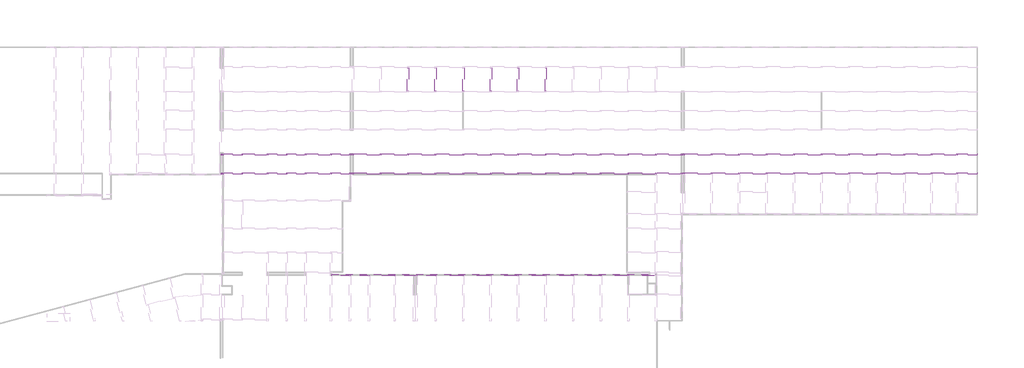
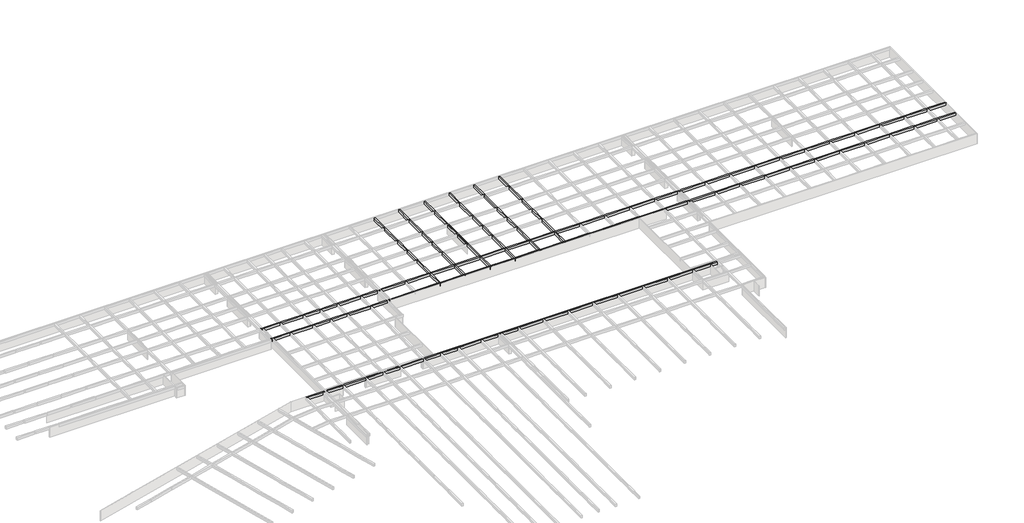
# One storey, part 11 of 14: 9 beams.
"""IFC4 building model written with IfcOpenShell, lengths in millimetres."""

from ifc_helpers import new_model, si_unit, frame, origin, place, context, project, spatial, polyline, outline, extrude, faceted_brep, element, save

model = new_model("IFC4")

# Units and contexts
model_context = context("Model", 3, world=origin())
ifc_project = project(units=[si_unit("LENGTHUNIT", "METRE", prefix="MILLI")], contexts=[model_context])

# Site, building, storey
site = spatial("IfcSite", under=ifc_project)
building = spatial("IfcBuilding", under=site)
storey = spatial("IfcBuildingStorey", under=building, Name="户型图", Elevation=0.0)

# Beams
placement = place(None, origin())
element("IfcBeam", 1, ObjectType="混凝土 - 矩形梁 : KL_beam", at=placement, inside=storey, context=model_context, shape_type="Brep", body=[
    faceted_brep([(227227.2949044, -147499.284307, 3300.0), (227227.2949044, -147899.284307, 3300.0), (227227.2949044, -147899.284307, 2500.0), (227227.2949044, -147499.284307, 2500.0), (221727.2949044, -147499.284307, 3300.0), (221327.2949044, -147499.284307, 3300.0), (214491.1566028, -147499.284307, 3300.0), (214091.1566028, -147499.284307, 3300.0), (206763.3308695, -147499.284307, 3300.0), (206363.3308695, -147499.284307, 3300.0), (198949.6658892, -147499.284307, 3300.0), (198549.6658892, -147499.284307, 3300.0), (191137.2949044, -147499.284307, 3300.0), (190737.2949044, -147499.284307, 3300.0), (183327.7006088, -147499.284307, 3300.0), (182927.7006088, -147499.284307, 3300.0), (175558.5232577, -147499.284307, 3300.0), (175158.5232577, -147499.284307, 3300.0), (167740.9658811, -147499.284307, 3300.0), (167340.9658811, -147499.284307, 3300.0), (159907.8874304, -147499.284307, 3300.0), (159507.8874304, -147499.284307, 3300.0), (152140.9658811, -147499.284307, 3300.0), (151740.9658811, -147499.284307, 3300.0), (144337.2949044, -147499.284307, 3300.0), (143937.2949044, -147499.284307, 3300.0), (143577.2949044, -147499.284307, 3300.0), (143177.2949044, -147499.284307, 3300.0), (136347.2949044, -147499.284307, 3300.0), (135947.2949044, -147499.284307, 3300.0), (128527.2949044, -147499.284307, 3300.0), (128127.2949044, -147499.284307, 3300.0), (120717.7893795, -147499.284307, 3300.0), (120317.7893795, -147499.284307, 3300.0), (112927.2949044, -147499.284307, 3300.0), (112527.2949044, -147499.284307, 3300.0), (105157.0968236, -147499.284307, 3300.0), (104757.0968236, -147499.284307, 3300.0), (97322.1026691, -147499.284307, 3300.0), (96922.1026691, -147499.284307, 3300.0), (89602.2949044, -147499.284307, 3300.0), (89202.2949044, -147499.284307, 3300.0), (81802.2949044, -147499.284307, 3300.0), (81402.2949044, -147499.284307, 3300.0), (73867.4871398, -147499.284307, 3300.0), (73467.4871398, -147499.284307, 3300.0), (66130.1134745, -147499.284307, 3300.0), (65730.1134745, -147499.284307, 3300.0), (58330.1134745, -147499.284307, 3300.0), (57930.1134745, -147499.284307, 3300.0), (50537.2949044, -147499.284307, 3300.0), (50137.2949044, -147499.284307, 3300.0), (49716.5330009, -147499.284307, 3300.0), (49316.5330009, -147499.284307, 3300.0), (44331.9066405, -147499.284307, 3300.0), (43931.9066405, -147499.284307, 3300.0), (37081.5607309, -147499.284307, 3300.0), (36681.5607309, -147499.284307, 3300.0), (31751.9066405, -147499.284307, 3300.0), (31351.9066405, -147499.284307, 3300.0), (26321.5607309, -147499.284307, 3300.0), (25921.5607309, -147499.284307, 3300.0), (19160.0865653, -147499.284307, 3300.0), (18760.0865653, -147499.284307, 3300.0), (13677.2949044, -147499.284307, 3300.0), (13277.2949044, -147499.284307, 3300.0), (12977.2949044, -147499.284307, 3300.0), (12977.2949044, -147899.284307, 3300.0), (13277.2949044, -147899.284307, 3300.0), (13677.2949044, -147899.284307, 3300.0), (18760.0865653, -147899.284307, 3300.0), (19160.0865653, -147899.284307, 3300.0), (25921.5607309, -147899.284307, 3300.0), (26321.5607309, -147899.284307, 3300.0), (31351.9066405, -147899.284307, 3300.0), (31751.9066405, -147899.284307, 3300.0), (36681.5607309, -147899.284307, 3300.0), (37081.5607309, -147899.284307, 3300.0), (43931.9066405, -147899.284307, 3300.0), (44331.9066405, -147899.284307, 3300.0), (49316.5330009, -147899.284307, 3300.0), (49716.5330009, -147899.284307, 3300.0), (50137.2949044, -147899.284307, 3300.0), (50537.2949044, -147899.284307, 3300.0), (57930.1134745, -147899.284307, 3300.0), (58330.1134745, -147899.284307, 3300.0), (65730.1134745, -147899.284307, 3300.0), (66130.1134745, -147899.284307, 3300.0), (73467.4871398, -147899.284307, 3300.0), (73867.4871398, -147899.284307, 3300.0), (81402.2949044, -147899.284307, 3300.0), (81802.2949044, -147899.284307, 3300.0), (89202.2949044, -147899.284307, 3300.0), (89602.2949044, -147899.284307, 3300.0), (96922.1026691, -147899.284307, 3300.0), (97322.1026691, -147899.284307, 3300.0), (104757.0968236, -147899.284307, 3300.0), (105157.0968236, -147899.284307, 3300.0), (112527.2949044, -147899.284307, 3300.0), (112927.2949044, -147899.284307, 3300.0), (120317.7893795, -147899.284307, 3300.0), (120717.7893795, -147899.284307, 3300.0), (128127.2949044, -147899.284307, 3300.0), (128527.2949044, -147899.284307, 3300.0), (135947.2949044, -147899.284307, 3300.0), (136347.2949044, -147899.284307, 3300.0), (143177.2949044, -147899.284307, 3300.0), (143577.2949044, -147899.284307, 3300.0), (143937.2949044, -147899.284307, 3300.0), (144337.2949044, -147899.284307, 3300.0), (151740.9658811, -147899.284307, 3300.0), (152140.9658811, -147899.284307, 3300.0), (159507.8874304, -147899.284307, 3300.0), (159907.8874304, -147899.284307, 3300.0), (167340.9658811, -147899.284307, 3300.0), (167740.9658811, -147899.284307, 3300.0), (175158.5232577, -147899.284307, 3300.0), (175558.5232577, -147899.284307, 3300.0), (182927.7006088, -147899.284307, 3300.0), (183327.7006088, -147899.284307, 3300.0), (190737.2949044, -147899.284307, 3300.0), (191137.2949044, -147899.284307, 3300.0), (198549.6658892, -147899.284307, 3300.0), (198949.6658892, -147899.284307, 3300.0), (206363.3308695, -147899.284307, 3300.0), (206763.3308695, -147899.284307, 3300.0), (214091.1566028, -147899.284307, 3300.0), (214491.1566028, -147899.284307, 3300.0), (221327.2949044, -147899.284307, 3300.0), (221727.2949044, -147899.284307, 3300.0), (12977.2949044, -147899.284307, 2500.0), (13277.2949044, -147899.284307, 2500.0), (13677.2949044, -147899.284307, 2500.0), (18760.0865653, -147899.284307, 2500.0), (19160.0865653, -147899.284307, 2500.0), (25921.5607309, -147899.284307, 2500.0), (26321.5607309, -147899.284307, 2500.0), (31351.9066405, -147899.284307, 2500.0), (31751.9066405, -147899.284307, 2500.0), (36681.5607309, -147899.284307, 2500.0), (37081.5607309, -147899.284307, 2500.0), (43931.9066405, -147899.284307, 2500.0), (44331.9066405, -147899.284307, 2500.0), (49316.5330009, -147899.284307, 2500.0), (49716.5330009, -147899.284307, 2500.0), (50137.2949044, -147899.284307, 2500.0), (50537.2949044, -147899.284307, 2500.0), (57930.1134745, -147899.284307, 2500.0), (58330.1134745, -147899.284307, 2500.0), (65730.1134745, -147899.284307, 2500.0), (66130.1134745, -147899.284307, 2500.0), (73467.4871398, -147899.284307, 2500.0), (73867.4871398, -147899.284307, 2500.0), (81402.2949044, -147899.284307, 2500.0), (81802.2949044, -147899.284307, 2500.0), (89202.2949044, -147899.284307, 2500.0), (89602.2949044, -147899.284307, 2500.0), (96922.1026691, -147899.284307, 2500.0), (97322.1026691, -147899.284307, 2500.0), (104757.0968236, -147899.284307, 2500.0), (105157.0968236, -147899.284307, 2500.0), (112527.2949044, -147899.284307, 2500.0), (112927.2949044, -147899.284307, 2500.0), (120317.7893795, -147899.284307, 2500.0), (120717.7893795, -147899.284307, 2500.0), (128127.2949044, -147899.284307, 2500.0), (128527.2949044, -147899.284307, 2500.0), (135947.2949044, -147899.284307, 2500.0), (136347.2949044, -147899.284307, 2500.0), (143177.2949044, -147899.284307, 2500.0), (143577.2949044, -147899.284307, 2500.0), (143937.2949044, -147899.284307, 2500.0), (144337.2949044, -147899.284307, 2500.0), (151740.9658811, -147899.284307, 2500.0), (152140.9658811, -147899.284307, 2500.0), (159507.8874304, -147899.284307, 2500.0), (159907.8874304, -147899.284307, 2500.0), (167340.9658811, -147899.284307, 2500.0), (167740.9658811, -147899.284307, 2500.0), (175158.5232577, -147899.284307, 2500.0), (175558.5232577, -147899.284307, 2500.0), (182927.7006088, -147899.284307, 2500.0), (183327.7006088, -147899.284307, 2500.0), (190737.2949044, -147899.284307, 2500.0), (191137.2949044, -147899.284307, 2500.0), (198549.6658892, -147899.284307, 2500.0), (198949.6658892, -147899.284307, 2500.0), (206363.3308695, -147899.284307, 2500.0), (206763.3308695, -147899.284307, 2500.0), (214091.1566028, -147899.284307, 2500.0), (214491.1566028, -147899.284307, 2500.0), (221327.2949044, -147899.284307, 2500.0), (221727.2949044, -147899.284307, 2500.0), (12977.2949044, -147499.284307, 2500.0), (13277.2949044, -147499.284307, 2500.0), (13677.2949044, -147499.284307, 2500.0), (18760.0865653, -147499.284307, 2500.0), (19160.0865653, -147499.284307, 2500.0), (25921.5607309, -147499.284307, 2500.0), (26321.5607309, -147499.284307, 2500.0), (31351.9066405, -147499.284307, 2500.0), (31751.9066405, -147499.284307, 2500.0), (36681.5607309, -147499.284307, 2500.0), (37081.5607309, -147499.284307, 2500.0), (43931.9066405, -147499.284307, 2500.0), (44331.9066405, -147499.284307, 2500.0), (49316.5330009, -147499.284307, 2500.0), (49716.5330009, -147499.284307, 2500.0), (50137.2949044, -147499.284307, 2500.0), (50537.2949044, -147499.284307, 2500.0), (57930.1134745, -147499.284307, 2500.0), (58330.1134745, -147499.284307, 2500.0), (65730.1134745, -147499.284307, 2500.0), (66130.1134745, -147499.284307, 2500.0), (73467.4871398, -147499.284307, 2500.0), (73867.4871398, -147499.284307, 2500.0), (81402.2949044, -147499.284307, 2500.0), (81802.2949044, -147499.284307, 2500.0), (89202.2949044, -147499.284307, 2500.0), (89602.2949044, -147499.284307, 2500.0), (96922.1026691, -147499.284307, 2500.0), (97322.1026691, -147499.284307, 2500.0), (104757.0968236, -147499.284307, 2500.0), (105157.0968236, -147499.284307, 2500.0), (112527.2949044, -147499.284307, 2500.0), (112927.2949044, -147499.284307, 2500.0), (120317.7893795, -147499.284307, 2500.0), (120717.7893795, -147499.284307, 2500.0), (128127.2949044, -147499.284307, 2500.0), (128527.2949044, -147499.284307, 2500.0), (135947.2949044, -147499.284307, 2500.0), (136347.2949044, -147499.284307, 2500.0), (143177.2949044, -147499.284307, 2500.0), (143577.2949044, -147499.284307, 2500.0), (143937.2949044, -147499.284307, 2500.0), (144337.2949044, -147499.284307, 2500.0), (151740.9658811, -147499.284307, 2500.0), (152140.9658811, -147499.284307, 2500.0), (159507.8874304, -147499.284307, 2500.0), (159907.8874304, -147499.284307, 2500.0), (167340.9658811, -147499.284307, 2500.0), (167740.9658811, -147499.284307, 2500.0), (175158.5232577, -147499.284307, 2500.0), (175558.5232577, -147499.284307, 2500.0), (182927.7006088, -147499.284307, 2500.0), (183327.7006088, -147499.284307, 2500.0), (190737.2949044, -147499.284307, 2500.0), (191137.2949044, -147499.284307, 2500.0), (198549.6658892, -147499.284307, 2500.0), (198949.6658892, -147499.284307, 2500.0), (206363.3308695, -147499.284307, 2500.0), (206763.3308695, -147499.284307, 2500.0), (214091.1566028, -147499.284307, 2500.0), (214491.1566028, -147499.284307, 2500.0), (221327.2949044, -147499.284307, 2500.0), (221727.2949044, -147499.284307, 2500.0)], [[[0, 1, 2, 3]], [[1, 0, 4, 5, 6, 7, 8, 9, 10, 11, 12, 13, 14, 15, 16, 17, 18, 19, 20, 21, 22, 23, 24, 25, 26, 27, 28, 29, 30, 31, 32, 33, 34, 35, 36, 37, 38, 39, 40, 41, 42, 43, 44, 45, 46, 47, 48, 49, 50, 51, 52, 53, 54, 55, 56, 57, 58, 59, 60, 61, 62, 63, 64, 65, 66, 67, 68, 69, 70, 71, 72, 73, 74, 75, 76, 77, 78, 79, 80, 81, 82, 83, 84, 85, 86, 87, 88, 89, 90, 91, 92, 93, 94, 95, 96, 97, 98, 99, 100, 101, 102, 103, 104, 105, 106, 107, 108, 109, 110, 111, 112, 113, 114, 115, 116, 117, 118, 119, 120, 121, 122, 123, 124, 125, 126, 127, 128, 129]], [[2, 1, 129, 128, 127, 126, 125, 124, 123, 122, 121, 120, 119, 118, 117, 116, 115, 114, 113, 112, 111, 110, 109, 108, 107, 106, 105, 104, 103, 102, 101, 100, 99, 98, 97, 96, 95, 94, 93, 92, 91, 90, 89, 88, 87, 86, 85, 84, 83, 82, 81, 80, 79, 78, 77, 76, 75, 74, 73, 72, 71, 70, 69, 68, 67, 130, 131, 132, 133, 134, 135, 136, 137, 138, 139, 140, 141, 142, 143, 144, 145, 146, 147, 148, 149, 150, 151, 152, 153, 154, 155, 156, 157, 158, 159, 160, 161, 162, 163, 164, 165, 166, 167, 168, 169, 170, 171, 172, 173, 174, 175, 176, 177, 178, 179, 180, 181, 182, 183, 184, 185, 186, 187, 188, 189, 190, 191, 192]], [[3, 2, 192, 191, 190, 189, 188, 187, 186, 185, 184, 183, 182, 181, 180, 179, 178, 177, 176, 175, 174, 173, 172, 171, 170, 169, 168, 167, 166, 165, 164, 163, 162, 161, 160, 159, 158, 157, 156, 155, 154, 153, 152, 151, 150, 149, 148, 147, 146, 145, 144, 143, 142, 141, 140, 139, 138, 137, 136, 135, 134, 133, 132, 131, 130, 193, 194, 195, 196, 197, 198, 199, 200, 201, 202, 203, 204, 205, 206, 207, 208, 209, 210, 211, 212, 213, 214, 215, 216, 217, 218, 219, 220, 221, 222, 223, 224, 225, 226, 227, 228, 229, 230, 231, 232, 233, 234, 235, 236, 237, 238, 239, 240, 241, 242, 243, 244, 245, 246, 247, 248, 249, 250, 251, 252, 253, 254, 255]], [[0, 3, 255, 254, 253, 252, 251, 250, 249, 248, 247, 246, 245, 244, 243, 242, 241, 240, 239, 238, 237, 236, 235, 234, 233, 232, 231, 230, 229, 228, 227, 226, 225, 224, 223, 222, 221, 220, 219, 218, 217, 216, 215, 214, 213, 212, 211, 210, 209, 208, 207, 206, 205, 204, 203, 202, 201, 200, 199, 198, 197, 196, 195, 194, 193, 66, 65, 64, 63, 62, 61, 60, 59, 58, 57, 56, 55, 54, 53, 52, 51, 50, 49, 48, 47, 46, 45, 44, 43, 42, 41, 40, 39, 38, 37, 36, 35, 34, 33, 32, 31, 30, 29, 28, 27, 26, 25, 24, 23, 22, 21, 20, 19, 18, 17, 16, 15, 14, 13, 12, 11, 10, 9, 8, 7, 6, 5, 4]], [[67, 66, 193, 130]]]),
])
element("IfcBeam", 2, ObjectType="混凝土 - 矩形梁 : KL_beam", at=placement, inside=storey, context=model_context, shape_type="Brep", body=[
    faceted_brep([(227227.2949044, -153299.284307, 3300.0), (227227.2949044, -153299.284307, 2500.0), (227227.2949044, -152899.284307, 2500.0), (227227.2949044, -152899.284307, 3300.0), (221727.2949044, -152899.284307, 3300.0), (221327.2949044, -152899.284307, 3300.0), (214491.1566028, -152899.284307, 3300.0), (214091.1566028, -152899.284307, 3300.0), (206763.3308695, -152899.284307, 3300.0), (206363.3308695, -152899.284307, 3300.0), (198949.6658892, -152899.284307, 3300.0), (198549.6658892, -152899.284307, 3300.0), (191137.2949044, -152899.284307, 3300.0), (190737.2949044, -152899.284307, 3300.0), (183327.7006088, -152899.284307, 3300.0), (182927.7006088, -152899.284307, 3300.0), (175558.5232577, -152899.284307, 3300.0), (175158.5232577, -152899.284307, 3300.0), (167740.9658811, -152899.284307, 3300.0), (167340.9658811, -152899.284307, 3300.0), (159907.8874304, -152899.284307, 3300.0), (159507.8874304, -152899.284307, 3300.0), (152140.9658811, -152899.284307, 3300.0), (151740.9658811, -152899.284307, 3300.0), (144337.2949044, -152899.284307, 3300.0), (143937.2949044, -152899.284307, 3300.0), (143577.2949044, -152899.284307, 3300.0), (143177.2949044, -152899.284307, 3300.0), (136347.2949044, -152899.284307, 3300.0), (135947.2949044, -152899.284307, 3300.0), (128527.2949044, -152899.284307, 3300.0), (128127.2949044, -152899.284307, 3300.0), (120717.7893795, -152899.284307, 3300.0), (120317.7893795, -152899.284307, 3300.0), (112927.2949044, -152899.284307, 3300.0), (112527.2949044, -152899.284307, 3300.0), (105157.0968236, -152899.284307, 3300.0), (104757.0968236, -152899.284307, 3300.0), (97322.1026691, -152899.284307, 3300.0), (96922.1026691, -152899.284307, 3300.0), (89602.2949044, -152899.284307, 3300.0), (89202.2949044, -152899.284307, 3300.0), (81802.2949044, -152899.284307, 3300.0), (81402.2949044, -152899.284307, 3300.0), (73867.4871398, -152899.284307, 3300.0), (73467.4871398, -152899.284307, 3300.0), (66130.1134745, -152899.284307, 3300.0), (65730.1134745, -152899.284307, 3300.0), (58330.1134745, -152899.284307, 3300.0), (57930.1134745, -152899.284307, 3300.0), (50537.2949044, -152899.284307, 3300.0), (50137.2949044, -152899.284307, 3300.0), (49716.5330009, -152899.284307, 3300.0), (49316.5330009, -152899.284307, 3300.0), (44331.9066405, -152899.284307, 3300.0), (43931.9066405, -152899.284307, 3300.0), (37081.5607309, -152899.284307, 3300.0), (36681.5607309, -152899.284307, 3300.0), (31751.9066405, -152899.284307, 3300.0), (31351.9066405, -152899.284307, 3300.0), (26321.5607309, -152899.284307, 3300.0), (25921.5607309, -152899.284307, 3300.0), (19160.0865653, -152899.284307, 3300.0), (18760.0865653, -152899.284307, 3300.0), (13677.2949044, -152899.284307, 3300.0), (13277.2949044, -152899.284307, 3300.0), (12977.2949044, -152899.284307, 3300.0), (12977.2949044, -153299.284307, 3300.0), (13277.2949044, -153299.284307, 3300.0), (13677.2949044, -153299.284307, 3300.0), (18760.0865653, -153299.284307, 3300.0), (19160.0865653, -153299.284307, 3300.0), (25921.5607309, -153299.284307, 3300.0), (26321.5607309, -153299.284307, 3300.0), (31351.9066405, -153299.284307, 3300.0), (31751.9066405, -153299.284307, 3300.0), (36681.5607309, -153299.284307, 3300.0), (37081.5607309, -153299.284307, 3300.0), (43931.9066405, -153299.284307, 3300.0), (44331.9066405, -153299.284307, 3300.0), (49316.5330009, -153299.284307, 3300.0), (49716.5330009, -153299.284307, 3300.0), (50137.2949044, -153299.284307, 3300.0), (50537.2949044, -153299.284307, 3300.0), (57930.1134745, -153299.284307, 3300.0), (58330.1134745, -153299.284307, 3300.0), (65730.1134745, -153299.284307, 3300.0), (66130.1134745, -153299.284307, 3300.0), (73467.4871398, -153299.284307, 3300.0), (73867.4871398, -153299.284307, 3300.0), (81402.2949044, -153299.284307, 3300.0), (81802.2949044, -153299.284307, 3300.0), (89202.2949044, -153299.284307, 3300.0), (89602.2949044, -153299.284307, 3300.0), (96922.1026691, -153299.284307, 3300.0), (97322.1026691, -153299.284307, 3300.0), (104757.0968236, -153299.284307, 3300.0), (105157.0968236, -153299.284307, 3300.0), (112527.2949044, -153299.284307, 3300.0), (112927.2949044, -153299.284307, 3300.0), (120317.7893795, -153299.284307, 3300.0), (120717.7893795, -153299.284307, 3300.0), (128127.2949044, -153299.284307, 3300.0), (128527.2949044, -153299.284307, 3300.0), (135947.2949044, -153299.284307, 3300.0), (136347.2949044, -153299.284307, 3300.0), (143177.2949044, -153299.284307, 3300.0), (143577.2949044, -153299.284307, 3300.0), (143937.2949044, -153299.284307, 3300.0), (144337.2949044, -153299.284307, 3300.0), (151740.9658811, -153299.284307, 3300.0), (152140.9658811, -153299.284307, 3300.0), (159507.8874304, -153299.284307, 3300.0), (159907.8874304, -153299.284307, 3300.0), (167340.9658811, -153299.284307, 3300.0), (167740.9658811, -153299.284307, 3300.0), (175158.5232577, -153299.284307, 3300.0), (175558.5232577, -153299.284307, 3300.0), (182927.7006088, -153299.284307, 3300.0), (183327.7006088, -153299.284307, 3300.0), (190737.2949044, -153299.284307, 3300.0), (191137.2949044, -153299.284307, 3300.0), (198549.6658892, -153299.284307, 3300.0), (198949.6658892, -153299.284307, 3300.0), (206363.3308695, -153299.284307, 3300.0), (206763.3308695, -153299.284307, 3300.0), (214091.1566028, -153299.284307, 3300.0), (214491.1566028, -153299.284307, 3300.0), (221327.2949044, -153299.284307, 3300.0), (221727.2949044, -153299.284307, 3300.0), (221727.2949044, -152899.284307, 2500.0), (221327.2949044, -152899.284307, 2500.0), (214491.1566028, -152899.284307, 2500.0), (214091.1566028, -152899.284307, 2500.0), (206763.3308695, -152899.284307, 2500.0), (206363.3308695, -152899.284307, 2500.0), (198949.6658892, -152899.284307, 2500.0), (198549.6658892, -152899.284307, 2500.0), (191137.2949044, -152899.284307, 2500.0), (190737.2949044, -152899.284307, 2500.0), (183327.7006088, -152899.284307, 2500.0), (182927.7006088, -152899.284307, 2500.0), (175558.5232577, -152899.284307, 2500.0), (175158.5232577, -152899.284307, 2500.0), (167740.9658811, -152899.284307, 2500.0), (167340.9658811, -152899.284307, 2500.0), (159907.8874304, -152899.284307, 2500.0), (159507.8874304, -152899.284307, 2500.0), (152140.9658811, -152899.284307, 2500.0), (151740.9658811, -152899.284307, 2500.0), (144337.2949044, -152899.284307, 2500.0), (143937.2949044, -152899.284307, 2500.0), (143577.2949044, -152899.284307, 2500.0), (143177.2949044, -152899.284307, 2500.0), (136347.2949044, -152899.284307, 2500.0), (135947.2949044, -152899.284307, 2500.0), (128527.2949044, -152899.284307, 2500.0), (128127.2949044, -152899.284307, 2500.0), (120717.7893795, -152899.284307, 2500.0), (120317.7893795, -152899.284307, 2500.0), (112927.2949044, -152899.284307, 2500.0), (112527.2949044, -152899.284307, 2500.0), (105157.0968236, -152899.284307, 2500.0), (104757.0968236, -152899.284307, 2500.0), (97322.1026691, -152899.284307, 2500.0), (96922.1026691, -152899.284307, 2500.0), (89602.2949044, -152899.284307, 2500.0), (89202.2949044, -152899.284307, 2500.0), (81802.2949044, -152899.284307, 2500.0), (81402.2949044, -152899.284307, 2500.0), (73867.4871398, -152899.284307, 2500.0), (73467.4871398, -152899.284307, 2500.0), (66130.1134745, -152899.284307, 2500.0), (65730.1134745, -152899.284307, 2500.0), (58330.1134745, -152899.284307, 2500.0), (57930.1134745, -152899.284307, 2500.0), (50537.2949044, -152899.284307, 2500.0), (50137.2949044, -152899.284307, 2500.0), (49716.5330009, -152899.284307, 2500.0), (49316.5330009, -152899.284307, 2500.0), (44331.9066405, -152899.284307, 2500.0), (43931.9066405, -152899.284307, 2500.0), (37081.5607309, -152899.284307, 2500.0), (36681.5607309, -152899.284307, 2500.0), (31751.9066405, -152899.284307, 2500.0), (31351.9066405, -152899.284307, 2500.0), (26321.5607309, -152899.284307, 2500.0), (25921.5607309, -152899.284307, 2500.0), (19160.0865653, -152899.284307, 2500.0), (18760.0865653, -152899.284307, 2500.0), (13677.2949044, -152899.284307, 2500.0), (13277.2949044, -152899.284307, 2500.0), (12977.2949044, -152899.284307, 2500.0), (221727.2949044, -153299.284307, 2500.0), (221327.2949044, -153299.284307, 2500.0), (214491.1566028, -153299.284307, 2500.0), (214091.1566028, -153299.284307, 2500.0), (206763.3308695, -153299.284307, 2500.0), (206363.3308695, -153299.284307, 2500.0), (198949.6658892, -153299.284307, 2500.0), (198549.6658892, -153299.284307, 2500.0), (191137.2949044, -153299.284307, 2500.0), (190737.2949044, -153299.284307, 2500.0), (183327.7006088, -153299.284307, 2500.0), (182927.7006088, -153299.284307, 2500.0), (175558.5232577, -153299.284307, 2500.0), (175158.5232577, -153299.284307, 2500.0), (167740.9658811, -153299.284307, 2500.0), (167340.9658811, -153299.284307, 2500.0), (159907.8874304, -153299.284307, 2500.0), (159507.8874304, -153299.284307, 2500.0), (152140.9658811, -153299.284307, 2500.0), (151740.9658811, -153299.284307, 2500.0), (144337.2949044, -153299.284307, 2500.0), (143937.2949044, -153299.284307, 2500.0), (143577.2949044, -153299.284307, 2500.0), (143177.2949044, -153299.284307, 2500.0), (136347.2949044, -153299.284307, 2500.0), (135947.2949044, -153299.284307, 2500.0), (128527.2949044, -153299.284307, 2500.0), (128127.2949044, -153299.284307, 2500.0), (120717.7893795, -153299.284307, 2500.0), (120317.7893795, -153299.284307, 2500.0), (112927.2949044, -153299.284307, 2500.0), (112527.2949044, -153299.284307, 2500.0), (105157.0968236, -153299.284307, 2500.0), (104757.0968236, -153299.284307, 2500.0), (97322.1026691, -153299.284307, 2500.0), (96922.1026691, -153299.284307, 2500.0), (89602.2949044, -153299.284307, 2500.0), (89202.2949044, -153299.284307, 2500.0), (81802.2949044, -153299.284307, 2500.0), (81402.2949044, -153299.284307, 2500.0), (73867.4871398, -153299.284307, 2500.0), (73467.4871398, -153299.284307, 2500.0), (66130.1134745, -153299.284307, 2500.0), (65730.1134745, -153299.284307, 2500.0), (58330.1134745, -153299.284307, 2500.0), (57930.1134745, -153299.284307, 2500.0), (50537.2949044, -153299.284307, 2500.0), (50137.2949044, -153299.284307, 2500.0), (49716.5330009, -153299.284307, 2500.0), (49316.5330009, -153299.284307, 2500.0), (44331.9066405, -153299.284307, 2500.0), (43931.9066405, -153299.284307, 2500.0), (37081.5607309, -153299.284307, 2500.0), (36681.5607309, -153299.284307, 2500.0), (31751.9066405, -153299.284307, 2500.0), (31351.9066405, -153299.284307, 2500.0), (26321.5607309, -153299.284307, 2500.0), (25921.5607309, -153299.284307, 2500.0), (19160.0865653, -153299.284307, 2500.0), (18760.0865653, -153299.284307, 2500.0), (13677.2949044, -153299.284307, 2500.0), (13277.2949044, -153299.284307, 2500.0), (12977.2949044, -153299.284307, 2500.0)], [[[0, 1, 2, 3]], [[0, 3, 4, 5, 6, 7, 8, 9, 10, 11, 12, 13, 14, 15, 16, 17, 18, 19, 20, 21, 22, 23, 24, 25, 26, 27, 28, 29, 30, 31, 32, 33, 34, 35, 36, 37, 38, 39, 40, 41, 42, 43, 44, 45, 46, 47, 48, 49, 50, 51, 52, 53, 54, 55, 56, 57, 58, 59, 60, 61, 62, 63, 64, 65, 66, 67, 68, 69, 70, 71, 72, 73, 74, 75, 76, 77, 78, 79, 80, 81, 82, 83, 84, 85, 86, 87, 88, 89, 90, 91, 92, 93, 94, 95, 96, 97, 98, 99, 100, 101, 102, 103, 104, 105, 106, 107, 108, 109, 110, 111, 112, 113, 114, 115, 116, 117, 118, 119, 120, 121, 122, 123, 124, 125, 126, 127, 128, 129]], [[3, 2, 130, 131, 132, 133, 134, 135, 136, 137, 138, 139, 140, 141, 142, 143, 144, 145, 146, 147, 148, 149, 150, 151, 152, 153, 154, 155, 156, 157, 158, 159, 160, 161, 162, 163, 164, 165, 166, 167, 168, 169, 170, 171, 172, 173, 174, 175, 176, 177, 178, 179, 180, 181, 182, 183, 184, 185, 186, 187, 188, 189, 190, 191, 192, 66, 65, 64, 63, 62, 61, 60, 59, 58, 57, 56, 55, 54, 53, 52, 51, 50, 49, 48, 47, 46, 45, 44, 43, 42, 41, 40, 39, 38, 37, 36, 35, 34, 33, 32, 31, 30, 29, 28, 27, 26, 25, 24, 23, 22, 21, 20, 19, 18, 17, 16, 15, 14, 13, 12, 11, 10, 9, 8, 7, 6, 5, 4]], [[2, 1, 193, 194, 195, 196, 197, 198, 199, 200, 201, 202, 203, 204, 205, 206, 207, 208, 209, 210, 211, 212, 213, 214, 215, 216, 217, 218, 219, 220, 221, 222, 223, 224, 225, 226, 227, 228, 229, 230, 231, 232, 233, 234, 235, 236, 237, 238, 239, 240, 241, 242, 243, 244, 245, 246, 247, 248, 249, 250, 251, 252, 253, 254, 255, 192, 191, 190, 189, 188, 187, 186, 185, 184, 183, 182, 181, 180, 179, 178, 177, 176, 175, 174, 173, 172, 171, 170, 169, 168, 167, 166, 165, 164, 163, 162, 161, 160, 159, 158, 157, 156, 155, 154, 153, 152, 151, 150, 149, 148, 147, 146, 145, 144, 143, 142, 141, 140, 139, 138, 137, 136, 135, 134, 133, 132, 131, 130]], [[1, 0, 129, 128, 127, 126, 125, 124, 123, 122, 121, 120, 119, 118, 117, 116, 115, 114, 113, 112, 111, 110, 109, 108, 107, 106, 105, 104, 103, 102, 101, 100, 99, 98, 97, 96, 95, 94, 93, 92, 91, 90, 89, 88, 87, 86, 85, 84, 83, 82, 81, 80, 79, 78, 77, 76, 75, 74, 73, 72, 71, 70, 69, 68, 67, 255, 254, 253, 252, 251, 250, 249, 248, 247, 246, 245, 244, 243, 242, 241, 240, 239, 238, 237, 236, 235, 234, 233, 232, 231, 230, 229, 228, 227, 226, 225, 224, 223, 222, 221, 220, 219, 218, 217, 216, 215, 214, 213, 212, 211, 210, 209, 208, 207, 206, 205, 204, 203, 202, 201, 200, 199, 198, 197, 196, 195, 194, 193]], [[67, 66, 192, 255]]]),
])
element("IfcBeam", 3, ObjectType="混凝土 - 矩形梁 : KL_beam", at=placement, inside=storey, context=model_context, shape_type="SweptSolid", body=[
    extrude(outline(polyline([(66130.1134745, -153358.950757), (65730.1134745, -153358.950757), (65730.1134745, -153299.284307), (66130.1134745, -153299.284307), (66130.1134745, -153358.950757)])), frame((0.0, 0.0, 2500.0), z_axis=(0.0, 0.0, 1.0), x_axis=(1.0, 0.0, 0.0)), (0.0, 0.0, 1.0), 800.0),
    extrude(outline(polyline([(65730.1134745, -123197.8127788), (66130.1134745, -123197.8127788), (66130.1134745, -129780.0179086), (65730.1134745, -129780.0179086), (65730.1134745, -123197.8127788)])), frame((0.0, 0.0, 2500.0), z_axis=(0.0, 0.0, 1.0), x_axis=(1.0, 0.0, 0.0)), (0.0, 0.0, 1.0), 800.0),
    extrude(outline(polyline([(66130.1134745, -122797.8127788), (65730.1134745, -122797.8127788), (65730.1134745, -117558.950757), (66130.1134745, -117558.950757), (66130.1134745, -122797.8127788)])), frame((0.0, 0.0, 2500.0), z_axis=(0.0, 0.0, 1.0), x_axis=(1.0, 0.0, 0.0)), (0.0, 0.0, 1.0), 800.0),
    extrude(outline(polyline([(65730.1134745, -130180.0179086), (66130.1134745, -130180.0179086), (66130.1134745, -135180.0179086), (65730.1134745, -135180.0179086), (65730.1134745, -130180.0179086)])), frame((0.0, 0.0, 2500.0), z_axis=(0.0, 0.0, 1.0), x_axis=(1.0, 0.0, 0.0)), (0.0, 0.0, 1.0), 800.0),
    extrude(outline(polyline([(65730.1134745, -135580.0179086), (66130.1134745, -135580.0179086), (66130.1134745, -140520.0179086), (65730.1134745, -140520.0179086), (65730.1134745, -135580.0179086)])), frame((0.0, 0.0, 2500.0), z_axis=(0.0, 0.0, 1.0), x_axis=(1.0, 0.0, 0.0)), (0.0, 0.0, 1.0), 800.0),
    extrude(outline(polyline([(65730.1134745, -140920.0179086), (66130.1134745, -140920.0179086), (66130.1134745, -147499.284307), (65730.1134745, -147499.284307), (65730.1134745, -140920.0179086)])), frame((0.0, 0.0, 2500.0), z_axis=(0.0, 0.0, 1.0), x_axis=(1.0, 0.0, 0.0)), (0.0, 0.0, 1.0), 800.0),
    extrude(outline(polyline([(65730.1134745, -147899.284307), (66130.1134745, -147899.284307), (66130.1134745, -152899.284307), (65730.1134745, -152899.284307), (65730.1134745, -147899.284307)])), frame((0.0, 0.0, 2500.0), z_axis=(0.0, 0.0, 1.0), x_axis=(1.0, 0.0, 0.0)), (0.0, 0.0, 1.0), 800.0),
])
element("IfcBeam", 4, ObjectType="混凝土 - 矩形梁 : KL_beam", at=placement, inside=storey, context=model_context, shape_type="SweptSolid", body=[
    extrude(outline(polyline([(73867.4871398, -153358.950757), (73467.4871398, -153358.950757), (73467.4871398, -153299.284307), (73867.4871398, -153299.284307), (73867.4871398, -153358.950757)])), frame((0.0, 0.0, 2500.0), z_axis=(0.0, 0.0, 1.0), x_axis=(1.0, 0.0, 0.0)), (0.0, 0.0, 1.0), 800.0),
    extrude(outline(polyline([(73467.4871398, -123197.8127788), (73867.4871398, -123197.8127788), (73867.4871398, -129780.0179086), (73467.4871398, -129780.0179086), (73467.4871398, -123197.8127788)])), frame((0.0, 0.0, 2500.0), z_axis=(0.0, 0.0, 1.0), x_axis=(1.0, 0.0, 0.0)), (0.0, 0.0, 1.0), 800.0),
    extrude(outline(polyline([(73867.4871398, -122797.8127788), (73467.4871398, -122797.8127788), (73467.4871398, -117558.950757), (73867.4871398, -117558.950757), (73867.4871398, -122797.8127788)])), frame((0.0, 0.0, 2500.0), z_axis=(0.0, 0.0, 1.0), x_axis=(1.0, 0.0, 0.0)), (0.0, 0.0, 1.0), 800.0),
    extrude(outline(polyline([(73467.4871398, -130180.0179086), (73867.4871398, -130180.0179086), (73867.4871398, -135180.0179086), (73467.4871398, -135180.0179086), (73467.4871398, -130180.0179086)])), frame((0.0, 0.0, 2500.0), z_axis=(0.0, 0.0, 1.0), x_axis=(1.0, 0.0, 0.0)), (0.0, 0.0, 1.0), 800.0),
    extrude(outline(polyline([(73467.4871398, -135580.0179086), (73867.4871398, -135580.0179086), (73867.4871398, -140520.0179086), (73467.4871398, -140520.0179086), (73467.4871398, -135580.0179086)])), frame((0.0, 0.0, 2500.0), z_axis=(0.0, 0.0, 1.0), x_axis=(1.0, 0.0, 0.0)), (0.0, 0.0, 1.0), 800.0),
    extrude(outline(polyline([(73467.4871398, -140920.0179086), (73867.4871398, -140920.0179086), (73867.4871398, -147499.284307), (73467.4871398, -147499.284307), (73467.4871398, -140920.0179086)])), frame((0.0, 0.0, 2500.0), z_axis=(0.0, 0.0, 1.0), x_axis=(1.0, 0.0, 0.0)), (0.0, 0.0, 1.0), 800.0),
    extrude(outline(polyline([(73467.4871398, -147899.284307), (73867.4871398, -147899.284307), (73867.4871398, -152899.284307), (73467.4871398, -152899.284307), (73467.4871398, -147899.284307)])), frame((0.0, 0.0, 2500.0), z_axis=(0.0, 0.0, 1.0), x_axis=(1.0, 0.0, 0.0)), (0.0, 0.0, 1.0), 800.0),
])
element("IfcBeam", 5, ObjectType="混凝土 - 矩形梁 : KL_beam", at=placement, inside=storey, context=model_context, shape_type="SweptSolid", body=[
    extrude(outline(polyline([(81802.2949044, -153358.950757), (81402.2949044, -153358.950757), (81402.2949044, -153299.284307), (81802.2949044, -153299.284307), (81802.2949044, -153358.950757)])), frame((0.0, 0.0, 2500.0), z_axis=(0.0, 0.0, 1.0), x_axis=(1.0, 0.0, 0.0)), (0.0, 0.0, 1.0), 800.0),
    extrude(outline(polyline([(81802.2949044, -122797.8127788), (81402.2949044, -122797.8127788), (81402.2949044, -117558.950757), (81802.2949044, -117558.950757), (81802.2949044, -122797.8127788)])), frame((0.0, 0.0, 2500.0), z_axis=(0.0, 0.0, 1.0), x_axis=(1.0, 0.0, 0.0)), (0.0, 0.0, 1.0), 800.0),
    extrude(outline(polyline([(81402.2949044, -123197.8127788), (81802.2949044, -123197.8127788), (81802.2949044, -129780.0179086), (81402.2949044, -129780.0179086), (81402.2949044, -123197.8127788)])), frame((0.0, 0.0, 2500.0), z_axis=(0.0, 0.0, 1.0), x_axis=(1.0, 0.0, 0.0)), (0.0, 0.0, 1.0), 800.0),
    extrude(outline(polyline([(81402.2949044, -130180.0179086), (81802.2949044, -130180.0179086), (81802.2949044, -135180.0179086), (81402.2949044, -135180.0179086), (81402.2949044, -130180.0179086)])), frame((0.0, 0.0, 2500.0), z_axis=(0.0, 0.0, 1.0), x_axis=(1.0, 0.0, 0.0)), (0.0, 0.0, 1.0), 800.0),
    extrude(outline(polyline([(81402.2949044, -135580.0179086), (81802.2949044, -135580.0179086), (81802.2949044, -140520.0179086), (81402.2949044, -140520.0179086), (81402.2949044, -135580.0179086)])), frame((0.0, 0.0, 2500.0), z_axis=(0.0, 0.0, 1.0), x_axis=(1.0, 0.0, 0.0)), (0.0, 0.0, 1.0), 800.0),
    extrude(outline(polyline([(81402.2949044, -140920.0179086), (81802.2949044, -140920.0179086), (81802.2949044, -147499.284307), (81402.2949044, -147499.284307), (81402.2949044, -140920.0179086)])), frame((0.0, 0.0, 2500.0), z_axis=(0.0, 0.0, 1.0), x_axis=(1.0, 0.0, 0.0)), (0.0, 0.0, 1.0), 800.0),
    extrude(outline(polyline([(81402.2949044, -147899.284307), (81802.2949044, -147899.284307), (81802.2949044, -152899.284307), (81402.2949044, -152899.284307), (81402.2949044, -147899.284307)])), frame((0.0, 0.0, 2500.0), z_axis=(0.0, 0.0, 1.0), x_axis=(1.0, 0.0, 0.0)), (0.0, 0.0, 1.0), 800.0),
])
element("IfcBeam", 6, ObjectType="混凝土 - 矩形梁 : KL_beam", at=placement, inside=storey, context=model_context, shape_type="SweptSolid", body=[
    extrude(outline(polyline([(89602.2949044, -153358.950757), (89202.2949044, -153358.950757), (89202.2949044, -153299.284307), (89602.2949044, -153299.284307), (89602.2949044, -153358.950757)])), frame((0.0, 0.0, 2500.0), z_axis=(0.0, 0.0, 1.0), x_axis=(1.0, 0.0, 0.0)), (0.0, 0.0, 1.0), 800.0),
    extrude(outline(polyline([(89202.2949044, -123197.8127788), (89602.2949044, -123197.8127788), (89602.2949044, -129780.0179086), (89202.2949044, -129780.0179086), (89202.2949044, -123197.8127788)])), frame((0.0, 0.0, 2500.0), z_axis=(0.0, 0.0, 1.0), x_axis=(1.0, 0.0, 0.0)), (0.0, 0.0, 1.0), 800.0),
    extrude(outline(polyline([(89602.2949044, -122797.8127788), (89202.2949044, -122797.8127788), (89202.2949044, -117558.950757), (89602.2949044, -117558.950757), (89602.2949044, -122797.8127788)])), frame((0.0, 0.0, 2500.0), z_axis=(0.0, 0.0, 1.0), x_axis=(1.0, 0.0, 0.0)), (0.0, 0.0, 1.0), 800.0),
    extrude(outline(polyline([(89202.2949044, -130180.0179086), (89602.2949044, -130180.0179086), (89602.2949044, -135180.0179086), (89202.2949044, -135180.0179086), (89202.2949044, -130180.0179086)])), frame((0.0, 0.0, 2500.0), z_axis=(0.0, 0.0, 1.0), x_axis=(1.0, 0.0, 0.0)), (0.0, 0.0, 1.0), 800.0),
    extrude(outline(polyline([(89202.2949044, -135580.0179086), (89602.2949044, -135580.0179086), (89602.2949044, -140520.0179086), (89202.2949044, -140520.0179086), (89202.2949044, -135580.0179086)])), frame((0.0, 0.0, 2500.0), z_axis=(0.0, 0.0, 1.0), x_axis=(1.0, 0.0, 0.0)), (0.0, 0.0, 1.0), 800.0),
    extrude(outline(polyline([(89202.2949044, -140920.0179086), (89602.2949044, -140920.0179086), (89602.2949044, -147499.284307), (89202.2949044, -147499.284307), (89202.2949044, -140920.0179086)])), frame((0.0, 0.0, 2500.0), z_axis=(0.0, 0.0, 1.0), x_axis=(1.0, 0.0, 0.0)), (0.0, 0.0, 1.0), 800.0),
    extrude(outline(polyline([(89202.2949044, -147899.284307), (89602.2949044, -147899.284307), (89602.2949044, -152899.284307), (89202.2949044, -152899.284307), (89202.2949044, -147899.284307)])), frame((0.0, 0.0, 2500.0), z_axis=(0.0, 0.0, 1.0), x_axis=(1.0, 0.0, 0.0)), (0.0, 0.0, 1.0), 800.0),
])
element("IfcBeam", 7, ObjectType="混凝土 - 矩形梁 : KL_beam", at=placement, inside=storey, context=model_context, shape_type="SweptSolid", body=[
    extrude(outline(polyline([(97322.1026691, -153358.950757), (96922.1026691, -153358.950757), (96922.1026691, -153299.284307), (97322.1026691, -153299.284307), (97322.1026691, -153358.950757)])), frame((0.0, 0.0, 2500.0), z_axis=(0.0, 0.0, 1.0), x_axis=(1.0, 0.0, 0.0)), (0.0, 0.0, 1.0), 800.0),
    extrude(outline(polyline([(97322.1026691, -122797.8127788), (96922.1026691, -122797.8127788), (96922.1026691, -117558.950757), (97322.1026691, -117558.950757), (97322.1026691, -122797.8127788)])), frame((0.0, 0.0, 2500.0), z_axis=(0.0, 0.0, 1.0), x_axis=(1.0, 0.0, 0.0)), (0.0, 0.0, 1.0), 800.0),
    extrude(outline(polyline([(96922.1026691, -123197.8127788), (97322.1026691, -123197.8127788), (97322.1026691, -129780.0179086), (96922.1026691, -129780.0179086), (96922.1026691, -123197.8127788)])), frame((0.0, 0.0, 2500.0), z_axis=(0.0, 0.0, 1.0), x_axis=(1.0, 0.0, 0.0)), (0.0, 0.0, 1.0), 800.0),
    extrude(outline(polyline([(96922.1026691, -130180.0179086), (97322.1026691, -130180.0179086), (97322.1026691, -135180.0179086), (96922.1026691, -135180.0179086), (96922.1026691, -130180.0179086)])), frame((0.0, 0.0, 2500.0), z_axis=(0.0, 0.0, 1.0), x_axis=(1.0, 0.0, 0.0)), (0.0, 0.0, 1.0), 800.0),
    extrude(outline(polyline([(96922.1026691, -135580.0179086), (97322.1026691, -135580.0179086), (97322.1026691, -140520.0179086), (96922.1026691, -140520.0179086), (96922.1026691, -135580.0179086)])), frame((0.0, 0.0, 2500.0), z_axis=(0.0, 0.0, 1.0), x_axis=(1.0, 0.0, 0.0)), (0.0, 0.0, 1.0), 800.0),
    extrude(outline(polyline([(96922.1026691, -140920.0179086), (97322.1026691, -140920.0179086), (97322.1026691, -147499.284307), (96922.1026691, -147499.284307), (96922.1026691, -140920.0179086)])), frame((0.0, 0.0, 2500.0), z_axis=(0.0, 0.0, 1.0), x_axis=(1.0, 0.0, 0.0)), (0.0, 0.0, 1.0), 800.0),
    extrude(outline(polyline([(96922.1026691, -147899.284307), (97322.1026691, -147899.284307), (97322.1026691, -152899.284307), (96922.1026691, -152899.284307), (96922.1026691, -147899.284307)])), frame((0.0, 0.0, 2500.0), z_axis=(0.0, 0.0, 1.0), x_axis=(1.0, 0.0, 0.0)), (0.0, 0.0, 1.0), 800.0),
])
element("IfcBeam", 8, ObjectType="混凝土 - 矩形梁 : KL_beam", at=placement, inside=storey, context=model_context, shape_type="SweptSolid", body=[
    extrude(outline(polyline([(105157.0968236, -153358.950757), (104757.0968236, -153358.950757), (104757.0968236, -153299.284307), (105157.0968236, -153299.284307), (105157.0968236, -153358.950757)])), frame((0.0, 0.0, 2500.0), z_axis=(0.0, 0.0, 1.0), x_axis=(1.0, 0.0, 0.0)), (0.0, 0.0, 1.0), 800.0),
    extrude(outline(polyline([(104757.0968236, -123197.8127788), (105157.0968236, -123197.8127788), (105157.0968236, -129780.0179086), (104757.0968236, -129780.0179086), (104757.0968236, -123197.8127788)])), frame((0.0, 0.0, 2500.0), z_axis=(0.0, 0.0, 1.0), x_axis=(1.0, 0.0, 0.0)), (0.0, 0.0, 1.0), 800.0),
    extrude(outline(polyline([(105157.0968236, -122797.8127788), (104757.0968236, -122797.8127788), (104757.0968236, -117558.950757), (105157.0968236, -117558.950757), (105157.0968236, -122797.8127788)])), frame((0.0, 0.0, 2500.0), z_axis=(0.0, 0.0, 1.0), x_axis=(1.0, 0.0, 0.0)), (0.0, 0.0, 1.0), 800.0),
    extrude(outline(polyline([(104757.0968236, -130180.0179086), (105157.0968236, -130180.0179086), (105157.0968236, -135180.0179086), (104757.0968236, -135180.0179086), (104757.0968236, -130180.0179086)])), frame((0.0, 0.0, 2500.0), z_axis=(0.0, 0.0, 1.0), x_axis=(1.0, 0.0, 0.0)), (0.0, 0.0, 1.0), 800.0),
    extrude(outline(polyline([(104757.0968236, -135580.0179086), (105157.0968236, -135580.0179086), (105157.0968236, -140520.0179086), (104757.0968236, -140520.0179086), (104757.0968236, -135580.0179086)])), frame((0.0, 0.0, 2500.0), z_axis=(0.0, 0.0, 1.0), x_axis=(1.0, 0.0, 0.0)), (0.0, 0.0, 1.0), 800.0),
    extrude(outline(polyline([(104757.0968236, -140920.0179086), (105157.0968236, -140920.0179086), (105157.0968236, -147499.284307), (104757.0968236, -147499.284307), (104757.0968236, -140920.0179086)])), frame((0.0, 0.0, 2500.0), z_axis=(0.0, 0.0, 1.0), x_axis=(1.0, 0.0, 0.0)), (0.0, 0.0, 1.0), 800.0),
    extrude(outline(polyline([(104757.0968236, -147899.284307), (105157.0968236, -147899.284307), (105157.0968236, -152899.284307), (104757.0968236, -152899.284307), (104757.0968236, -147899.284307)])), frame((0.0, 0.0, 2500.0), z_axis=(0.0, 0.0, 1.0), x_axis=(1.0, 0.0, 0.0)), (0.0, 0.0, 1.0), 800.0),
])
element("IfcBeam", 9, ObjectType="混凝土 - 矩形梁 : KL_beam", at=placement, inside=storey, context=model_context, shape_type="Brep", body=[
    faceted_brep([(7447.2949044, -182068.950757, 3300.0), (7447.2949044, -181668.950757, 3300.0), (7447.2949044, -181668.950757, 2500.0), (7447.2949044, -182068.950757, 2500.0), (7722.5700952, -182068.950757, 3300.0), (12533.1378826, -182068.950757, 3300.0), (12933.1378826, -182068.950757, 3300.0), (13377.4621399, -182068.950757, 3300.0), (13777.4621399, -182068.950757, 3300.0), (18760.0865653, -182068.950757, 3300.0), (19160.0865653, -182068.950757, 3300.0), (25921.5607309, -182068.950757, 3300.0), (25921.5607309, -181668.950757, 3300.0), (19160.0865653, -181668.950757, 3300.0), (18760.0865653, -181668.950757, 3300.0), (13677.2949044, -181668.950757, 3300.0), (13277.2949044, -181668.950757, 3300.0), (7722.5700952, -181668.950757, 3300.0), (25921.5607309, -181668.950757, 2500.0), (19160.0865653, -181668.950757, 2500.0), (18760.0865653, -181668.950757, 2500.0), (13677.2949044, -181668.950757, 2500.0), (13277.2949044, -181668.950757, 2500.0), (7722.5700952, -181668.950757, 2500.0), (25921.5607309, -182068.950757, 2500.0), (19160.0865653, -182068.950757, 2500.0), (18760.0865653, -182068.950757, 2500.0), (13777.4621399, -182068.950757, 2500.0), (13377.4621399, -182068.950757, 2500.0), (12933.1378826, -182068.950757, 2500.0), (12533.1378826, -182068.950757, 2500.0), (7722.5700952, -182068.950757, 2500.0)], [[[0, 1, 2, 3]], [[1, 0, 4, 5, 6, 7, 8, 9, 10, 11, 12, 13, 14, 15, 16, 17]], [[2, 1, 17, 16, 15, 14, 13, 12, 18, 19, 20, 21, 22, 23]], [[3, 2, 23, 22, 21, 20, 19, 18, 24, 25, 26, 27, 28, 29, 30, 31]], [[0, 3, 31, 30, 29, 28, 27, 26, 25, 24, 11, 10, 9, 8, 7, 6, 5, 4]], [[12, 11, 24, 18]]]),
    faceted_brep([(135947.2949044, -181668.950757, 3300.0), (135947.2949044, -182068.950757, 3300.0), (135947.2949044, -182068.950757, 2500.0), (135947.2949044, -181668.950757, 2500.0), (44331.9066405, -182068.950757, 3300.0), (44331.9066405, -181668.950757, 3300.0), (44331.9066405, -181668.950757, 2500.0), (44331.9066405, -182068.950757, 2500.0), (49289.9831968, -182068.950757, 3300.0), (49689.9831968, -182068.950757, 3300.0), (54689.9831968, -182068.950757, 3300.0), (55089.9831968, -182068.950757, 3300.0), (61967.2949044, -182068.950757, 3300.0), (62367.2949044, -182068.950757, 3300.0), (67367.2949044, -182068.950757, 3300.0), (67767.2949044, -182068.950757, 3300.0), (68177.2949044, -182068.950757, 3300.0), (68577.2949044, -182068.950757, 3300.0), (73579.8514216, -182068.950757, 3300.0), (73979.8514216, -182068.950757, 3300.0), (81379.8514216, -182068.950757, 3300.0), (81779.8514216, -182068.950757, 3300.0), (89134.3329203, -182068.950757, 3300.0), (89534.3329203, -182068.950757, 3300.0), (96934.3329203, -182068.950757, 3300.0), (97334.3329203, -182068.950757, 3300.0), (104734.3329203, -182068.950757, 3300.0), (105134.3329203, -182068.950757, 3300.0), (112555.6695954, -182068.950757, 3300.0), (112955.6695954, -182068.950757, 3300.0), (120367.2949044, -182068.950757, 3300.0), (120767.2949044, -182068.950757, 3300.0), (128149.172254, -182068.950757, 3300.0), (128549.172254, -182068.950757, 3300.0), (128549.172254, -182068.950757, 2500.0), (128149.172254, -182068.950757, 2500.0), (120767.2949044, -182068.950757, 2500.0), (120367.2949044, -182068.950757, 2500.0), (112955.6695954, -182068.950757, 2500.0), (112555.6695954, -182068.950757, 2500.0), (105134.3329203, -182068.950757, 2500.0), (104734.3329203, -182068.950757, 2500.0), (97334.3329203, -182068.950757, 2500.0), (96934.3329203, -182068.950757, 2500.0), (89534.3329203, -182068.950757, 2500.0), (89134.3329203, -182068.950757, 2500.0), (81779.8514216, -182068.950757, 2500.0), (81379.8514216, -182068.950757, 2500.0), (73979.8514216, -182068.950757, 2500.0), (73579.8514216, -182068.950757, 2500.0), (68577.2949044, -182068.950757, 2500.0), (68177.2949044, -182068.950757, 2500.0), (67767.2949044, -182068.950757, 2500.0), (67367.2949044, -182068.950757, 2500.0), (62367.2949044, -182068.950757, 2500.0), (61967.2949044, -182068.950757, 2500.0), (55089.9831968, -182068.950757, 2500.0), (54689.9831968, -182068.950757, 2500.0), (49689.9831968, -182068.950757, 2500.0), (49289.9831968, -182068.950757, 2500.0)], [[[0, 1, 2, 3]], [[4, 5, 6, 7]], [[1, 0, 5, 4, 8, 9, 10, 11, 12, 13, 14, 15, 16, 17, 18, 19, 20, 21, 22, 23, 24, 25, 26, 27, 28, 29, 30, 31, 32, 33]], [[0, 3, 6, 5]], [[3, 2, 34, 35, 36, 37, 38, 39, 40, 41, 42, 43, 44, 45, 46, 47, 48, 49, 50, 51, 52, 53, 54, 55, 56, 57, 58, 59, 7, 6]], [[2, 1, 33, 32, 31, 30, 29, 28, 27, 26, 25, 24, 23, 22, 21, 20, 19, 18, 17, 16, 15, 14, 13, 12, 11, 10, 9, 8, 4, 7, 59, 58, 57, 56, 55, 54, 53, 52, 51, 50, 49, 48, 47, 46, 45, 44, 43, 42, 41, 40, 39, 38, 37, 36, 35, 34]]]),
    faceted_brep([(26321.5607309, -182068.950757, 3300.0), (26321.5607309, -181668.950757, 3300.0), (26321.5607309, -181668.950757, 2500.0), (26321.5607309, -182068.950757, 2500.0), (31351.9066405, -182068.950757, 3300.0), (31351.9066405, -181668.950757, 3300.0), (31351.9066405, -181668.950757, 2500.0), (31351.9066405, -182068.950757, 2500.0)], [[[0, 1, 2, 3]], [[1, 0, 4, 5]], [[2, 1, 5, 6]], [[3, 2, 6, 7]], [[0, 3, 7, 4]], [[5, 4, 7, 6]]]),
    faceted_brep([(31751.9066405, -182068.950757, 3300.0), (31751.9066405, -181668.950757, 3300.0), (31751.9066405, -181668.950757, 2500.0), (31751.9066405, -182068.950757, 2500.0), (36681.5607309, -182068.950757, 3300.0), (36681.5607309, -181668.950757, 3300.0), (36681.5607309, -181668.950757, 2500.0), (36681.5607309, -182068.950757, 2500.0)], [[[0, 1, 2, 3]], [[1, 0, 4, 5]], [[2, 1, 5, 6]], [[3, 2, 6, 7]], [[0, 3, 7, 4]], [[5, 4, 7, 6]]]),
    faceted_brep([(37081.5607309, -182068.950757, 3300.0), (37081.5607309, -181668.950757, 3300.0), (37081.5607309, -181668.950757, 2500.0), (37081.5607309, -182068.950757, 2500.0), (43931.9066405, -182068.950757, 3300.0), (43931.9066405, -181668.950757, 3300.0), (43931.9066405, -181668.950757, 2500.0), (43931.9066405, -182068.950757, 2500.0)], [[[0, 1, 2, 3]], [[1, 0, 4, 5]], [[2, 1, 5, 6]], [[3, 2, 6, 7]], [[0, 3, 7, 4]], [[5, 4, 7, 6]]]),
])

save(model, "model.ifc")

# Revit data of these elements
# Type "混凝土 - 矩形梁 : KL_beam"
#   Length [instance default] = 1524 mm
#   b = 400 mm
#   h = 800 mm
#   Structural Material [instance default] = 混凝土 - 现场浇注混凝土
#   Assembly Code = ""
# Elements 1, 2, 3, 4, 5, 6, 7, 8, 9 (IfcBeam, "混凝土 - 矩形梁 : KL_beam")
#   Comments = ""
#   Structural Material = none
#   Phase Created = 新构造
# Materials
#   "混凝土 - 现场浇注混凝土": class "混凝土", colour RGB 192 192 192, transparency 0
